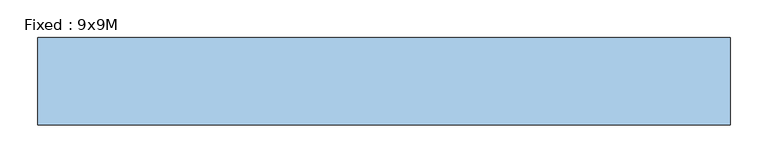
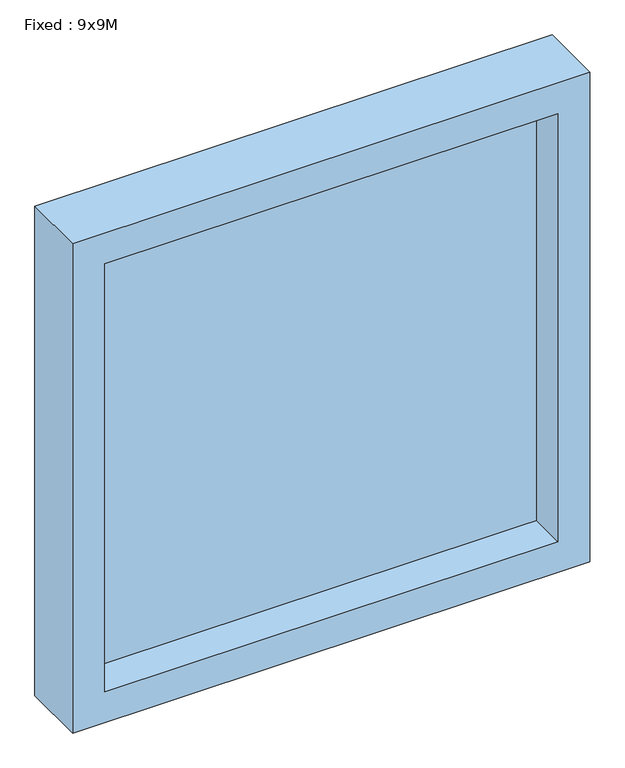
"""IFC4 building model written with IfcOpenShell, lengths in millimetres: window geometry, Fixed : 9x9M."""

import ifcopenshell
import ifcopenshell.guid

model = None  # the IFC model being written
_history = None  # IfcOwnerHistory: only IFC2X3 demands one
_inside = {}  # id of a spatial element -> (the spatial element, [elements in it])
_under = {}  # id of a project, library or spatial element -> (it, [spatial elements below it])
_declared = {}  # id of a project -> (the project, [libraries it declares])
_typed = {}  # id of a type object -> (the type object, [elements of that type])
_made_of = {}  # id of a material, layer set ... -> (it, [elements and type objects made of it])


def new_model(schema):
    """Start an empty IFC model of exactly this schema.

    Asked for "IFC4X3", IfcOpenShell would pick the latest addendum, in which some entities
    have other attributes; the version numbers below select the first issue.
    IFC2X3 requires an IfcOwnerHistory on every rooted entity: one is made here for all.
    """
    global model, _history
    if schema == "IFC4X3":
        model = ifcopenshell.file(schema_version=(4, 3, 0, 0))
    else:
        model = ifcopenshell.file(schema=schema)
    _inside.clear()
    _under.clear()
    _declared.clear()
    _typed.clear()
    _made_of.clear()
    _history = None
    if model.schema == "IFC2X3":
        org = make("IfcOrganization", Name="unknown")
        user = make(
            "IfcPersonAndOrganization",
            ThePerson=make("IfcPerson", FamilyName="unknown"),
            TheOrganization=org,
        )
        app = make(
            "IfcApplication",
            ApplicationDeveloper=org,
            Version="unknown",
            ApplicationFullName="unknown",
            ApplicationIdentifier="unknown",
        )
        _history = make(
            "IfcOwnerHistory",
            OwningUser=user,
            OwningApplication=app,
            ChangeAction="ADDED",
            CreationDate=0,
        )
    return model


def make(cls, **values):
    """One entity of the class cls with the attributes given. An attribute that is None is left unset."""
    return model.create_entity(
        cls, **{name: value for name, value in values.items() if value is not None}
    )


def rooted(cls, **values):
    """An entity with a GlobalId (a new one), such as an element, a storey or a relation."""
    return make(cls, GlobalId=ifcopenshell.guid.new(), OwnerHistory=_history, **values)


def si_unit(unit_type, name, prefix=None):
    """IfcSIUnit, for example si_unit("LENGTHUNIT", "METRE", prefix="MILLI")."""
    return make("IfcSIUnit", UnitType=unit_type, Prefix=prefix, Name=name)


def assignment(units):
    """IfcUnitAssignment: the units of a project."""
    return None if units is None else make("IfcUnitAssignment", Units=units)


def point(xyz):
    """IfcCartesianPoint."""
    return None if xyz is None else make("IfcCartesianPoint", Coordinates=xyz)


def direction(xyz):
    """IfcDirection."""
    return None if xyz is None else make("IfcDirection", DirectionRatios=xyz)


def frame(location, z_axis=None, x_axis=None):
    """IfcAxis2Placement3D, a coordinate frame: its origin and axes. An axis left out is left unset."""
    return make(
        "IfcAxis2Placement3D",
        Location=point(location),
        Axis=direction(z_axis),
        RefDirection=direction(x_axis),
    )


def origin():
    """The frame at (0, 0, 0) with its axes left unset."""
    return frame((0.0, 0.0, 0.0))


def place(relative_to, where):
    """IfcLocalPlacement: puts the frame where relative to a parent placement (None: the world)."""
    return make(
        "IfcLocalPlacement", PlacementRelTo=relative_to, RelativePlacement=where
    )


def context(
    kind, dimensions, precision=None, world=None, true_north=None, identifier=None
):
    """IfcGeometricRepresentationContext, for example the 3D "Model" context."""
    return make(
        "IfcGeometricRepresentationContext",
        ContextIdentifier=identifier,
        ContextType=kind,
        CoordinateSpaceDimension=dimensions,
        Precision=precision,
        WorldCoordinateSystem=world,
        TrueNorth=true_north,
    )


def project(units=None, contexts=None):
    """IfcProject with its units and contexts."""
    return rooted(
        "IfcProject",
        Name="project",
        RepresentationContexts=contexts,
        UnitsInContext=assignment(units),
    )


def spatial(cls, under=None, at=None, **own):
    """A site, building, storey or space (cls), placed at a placement, below another one or the project."""
    s = rooted(cls, ObjectPlacement=at, **own)
    if under is not None:
        _under.setdefault(under.id(), (under, []))[1].append(s)
    return s


def polyline(points):
    """IfcPolyline through the points."""
    return make("IfcPolyline", Points=[point(p) for p in points])


def outline(outer, holes=None, kind="AREA"):
    """IfcArbitraryClosedProfileDef: a profile drawn as a closed curve; with holes, ...WithVoids."""
    if holes is None:
        return make("IfcArbitraryClosedProfileDef", ProfileType=kind, OuterCurve=outer)
    return make(
        "IfcArbitraryProfileDefWithVoids",
        ProfileType=kind,
        OuterCurve=outer,
        InnerCurves=holes,
    )


def extrude(swept, where, along, depth):
    """IfcExtrudedAreaSolid: the profile swept, set in the frame where, extruded along a direction by depth."""
    return make(
        "IfcExtrudedAreaSolid",
        SweptArea=swept,
        Position=where,
        ExtrudedDirection=direction(along),
        Depth=depth,
    )


def shape(context_of_items, identifier, shape_type, items):
    """IfcShapeRepresentation: the items that make up one representation, for example the "Body"."""
    return make(
        "IfcShapeRepresentation",
        ContextOfItems=context_of_items,
        RepresentationIdentifier=identifier,
        RepresentationType=shape_type,
        Items=items,
    )


def source(mapping_origin, context_of_items, identifier, shape_type, items):
    """IfcRepresentationMap: a shape defined once, which mapped items show again and again."""
    return make(
        "IfcRepresentationMap",
        MappingOrigin=mapping_origin,
        MappedRepresentation=shape(context_of_items, identifier, shape_type, items),
    )


def transform(
    local_origin,
    x_axis=None,
    y_axis=None,
    z_axis=None,
    scale=None,
    scale2=None,
    scale3=None,
    uniform=True,
):
    """IfcCartesianTransformationOperator3D, or its non-uniform kind. x_axis, y_axis, z_axis: its Axis1, 2, 3."""
    if uniform:
        return make(
            "IfcCartesianTransformationOperator3D",
            Axis1=direction(x_axis),
            Axis2=direction(y_axis),
            LocalOrigin=point(local_origin),
            Scale=scale,
            Axis3=direction(z_axis),
        )
    return make(
        "IfcCartesianTransformationOperator3DnonUniform",
        Axis1=direction(x_axis),
        Axis2=direction(y_axis),
        LocalOrigin=point(local_origin),
        Scale=scale,
        Axis3=direction(z_axis),
        Scale2=scale2,
        Scale3=scale3,
    )


def mapped(mapping_source, mapping_target):
    """IfcMappedItem: shows the shape of a source again, moved by a transform."""
    return make(
        "IfcMappedItem", MappingSource=mapping_source, MappingTarget=mapping_target
    )


def made_of(thing, what):
    """Note that an element or type object is made of a material, layer set ...; save() writes the relation."""
    if what is not None:
        _made_of.setdefault(what.id(), (what, []))[1].append(thing)
    return thing


def element(
    cls,
    number,
    at=None,
    inside=None,
    cuts=None,
    type_object=None,
    material=None,
    context=None,
    identifier="Body",
    shape_type=None,
    held_by="IfcProductDefinitionShape",
    body=None,
    shapes=None,
    **own,
):
    """One element of the class cls, such as IfcWall. Its Tag is "e" and its number.

    at: its placement. inside: the storey or other place that contains it. cuts: it is an
    opening in that element (IfcRelVoidsElement). A single representation is given by context,
    identifier, shape_type and body (its items); several are given by shapes. held_by: the class
    of the entity that holds the representations. save() writes the other relations.
    """
    e = rooted(cls, Tag="e%d" % number, ObjectPlacement=at, **own)
    if body is not None:
        shapes = [shape(context, identifier, shape_type, body)]
    if shapes is not None:
        e.Representation = make(held_by, Representations=shapes)
    if inside is not None:
        _inside.setdefault(inside.id(), (inside, []))[1].append(e)
    if cuts is not None:
        rooted(
            "IfcRelVoidsElement", RelatingBuildingElement=cuts, RelatedOpeningElement=e
        )
    if type_object is not None:
        _typed.setdefault(type_object.id(), (type_object, []))[1].append(e)
    return made_of(e, material)


def aggregate(whole, parts):
    """IfcRelAggregates: a whole, such as a stair, and the parts it consists of."""
    return rooted("IfcRelAggregates", RelatingObject=whole, RelatedObjects=parts)


def save(model, path):
    """Write the relations noted so far, then the file.

    IfcRelAggregates (storeys below a building ...), IfcRelContainedInSpatialStructure (elements
    in a storey), IfcRelDefinesByType, IfcRelAssociatesMaterial and IfcRelDeclares: one each for
    every whole, place, type object, material and project.
    """
    for whole, parts in _under.values():
        aggregate(whole, parts)
    for where, things in _inside.values():
        rooted(
            "IfcRelContainedInSpatialStructure",
            RelatedElements=things,
            RelatingStructure=where,
        )
    for kind, things in _typed.values():
        rooted("IfcRelDefinesByType", RelatedObjects=things, RelatingType=kind)
    for what, things in _made_of.values():
        rooted("IfcRelAssociatesMaterial", RelatedObjects=things, RelatingMaterial=what)
    for by, libraries in _declared.values():
        rooted("IfcRelDeclares", RelatingContext=by, RelatedDefinitions=libraries)
    model.write(path)


def fixed_9x9m_da96294a(model_context):
    return source(origin(), model_context, "Body", "SweptSolid", [
        extrude(outline(polyline([(1712.0, 456.0), (1712.0, -456.0), (800.0, -456.0), (800.0, 456.0), (1712.0, 456.0)]), holes=[polyline([(857.0, 399.0), (857.0, -399.0), (1655.0, -399.0), (1655.0, 399.0), (857.0, 399.0)])]), frame((0.0, 69.0, 0.0), z_axis=(0.0, 1.0, 0.0), x_axis=(0.0, 0.0, 1.0)), (0.0, 0.0, 1.0), 115.0),
        extrude(outline(polyline([(-399.0, 162.0), (399.0, 162.0), (399.0, 134.0), (-399.0, 134.0), (-399.0, 162.0)])), frame((0.0, 0.0, 857.0), z_axis=(0.0, 0.0, 1.0), x_axis=(1.0, 0.0, 0.0)), (0.0, 0.0, 1.0), 798.0),
    ])


if __name__ == "__main__":
    model = new_model("IFC4")
    model_context = context("Model", 3, world=origin())
    ifc_project = project(units=[si_unit("LENGTHUNIT", "METRE", prefix="MILLI")], contexts=[model_context])
    site = spatial("IfcSite", under=ifc_project)
    building = spatial("IfcBuilding", under=site)
    placement = place(None, origin())
    fixed_9x9m_shape = fixed_9x9m_da96294a(model_context)
    element("IfcWindow", 1, ObjectType="Fixed : 9x9M", at=placement, inside=building, context=model_context, shape_type="MappedRepresentation", body=[
        mapped(fixed_9x9m_shape, transform((0.0, 0.0, 0.0), x_axis=(1.0, 0.0, 0.0), y_axis=(0.0, 1.0, 0.0), z_axis=(0.0, 0.0, 1.0))),
    ])
    save(model, "model.ifc")

# Revit data of these elements
# Project information
#   Client Name = "Test Project"
#   Project Address = "Enter address here"
#   Project Number = "Number"
#   Current Version = "0.0.0"
#   SR Document GUID = "3eb9317e-835d-4f79-8926-4d15b96bc824"
# Type "Fixed : 9x9M"
#   Type Mark = "46"
#   Creator Organization [instance default] = "© Danish Educational Content"
#   Creator Name [instance default] = "© Erik Falck Jørgensen"
#   Creator Build [instance default] = "2017.0801.0"
#   Analytic Construction = "<None>"
#   length#5 = -22 mm
#   length#4 = -50 mm
#   length#3 = 100 mm
#   length#2 = 57 mm
#   length#1 = 0 mm
#   Seal Width = 12 mm
#   Rough Width = 912 mm
#   Rough Height = 912 mm
#   Rebate Depth = 50 mm
#   Height = 888 mm
#   Glass Thickness = 28 mm
#   Exterior Direction [instance default] = 0.00°
#   Default Sill Height = 800 mm
#   Width = 888 mm
#   Case Width = 45 mm
#   Case Depth = 115 mm
#   Sealing = no
#   Wall Closure = 1
#   Above Cutplane [instance default] = no
#   Wall Surface = none
#   Sill Plate = none
#   Glass = none
#   Embrasure = none
#   Case/Transom = none
#   Assembly Code = ""
# Element 1 (IfcWindow, "Fixed : 9x9M")
#   Materials on its faces: "Default Frame/Mullion (Interior/Exterior)", "Glass"
# Materials
#   "Default Frame/Mullion (Interior/Exterior)": class "Generic", colour RGB 205 205 205, transparency 0, Description = "Udefineret karm/ramme materiale", Cost = 0
#   "Glass": class "Glass", colour RGB 180 200 255, transparency 0.75, Description = "Generisk glas", Cost = 0
